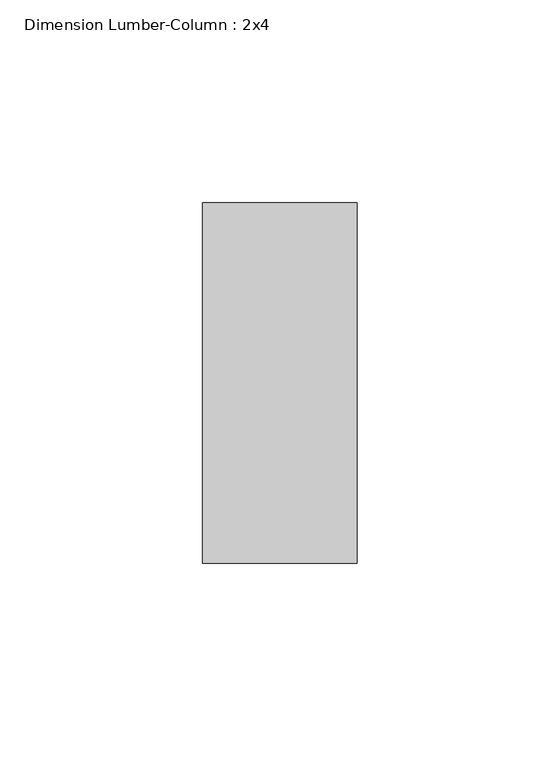
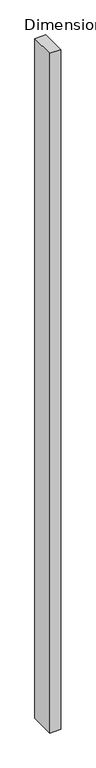
"""IFC4 building model written with IfcOpenShell, lengths in millimetres: column geometry, Dimension Lumber-Column : 2x4."""

from ifc_helpers import new_model, si_unit, frame, origin, place, context, project, spatial, polyline, outline, extrude, source, transform, mapped, element, save


def dimension_lumber_column_2x4_3536d246(model_context):
    return source(origin(), model_context, "Body", "SweptSolid", [
        extrude(outline(polyline([(19.05, 44.45), (19.05, -44.45), (-19.05, -44.45), (-19.05, 44.45), (19.05, 44.45)])), frame((0.0, 0.0, 56.35625), z_axis=(0.0, 0.0, 1.0), x_axis=(1.0, 0.0, 0.0)), (0.0, 0.0, 1.0), 2477.29375),
    ])


if __name__ == "__main__":
    model = new_model("IFC4")
    model_context = context("Model", 3, world=origin())
    ifc_project = project(units=[si_unit("LENGTHUNIT", "METRE", prefix="MILLI")], contexts=[model_context])
    site = spatial("IfcSite", under=ifc_project)
    building = spatial("IfcBuilding", under=site)
    placement = place(None, origin())
    dimension_lumber_column_2x4_shape = dimension_lumber_column_2x4_3536d246(model_context)
    element("IfcColumn", 1, ObjectType="Dimension Lumber-Column : 2x4", at=placement, inside=building, context=model_context, shape_type="MappedRepresentation", body=[
        mapped(dimension_lumber_column_2x4_shape, transform((0.0, 0.0, 0.0), x_axis=(1.0, 0.0, 0.0), y_axis=(0.0, 1.0, 0.0), z_axis=(0.0, 0.0, 1.0))),
    ])
    save(model, "model.ifc")

# Revit data of these elements
# Type "Dimension Lumber-Column : 2x4"
#   Int Type = "Interior"
#   Assembly Code = "B10"
#   Cost = 8.05
#   A = 0.0364583 SF
#   b = 0' - 1 1/2"
#   d = 0' - 3 1/2"
#   Structural Material [instance default] = Softwood, Lumber
# Element 1 (IfcColumn, "Dimension Lumber-Column : 2x4")
#   Structural Material = Douglas Fir #2
#   Materials on its faces: "Douglas Fir #2"
# Materials
#   "Softwood, Lumber": class "Wood", colour RGB 223 192 134, transparency 0, Description = "Pinus Echinata", Cost = 0
#   "Douglas Fir #2": class "Wood", colour RGB 223 192 134, transparency 0, Description = "Pinus Echinata", Cost = 0
